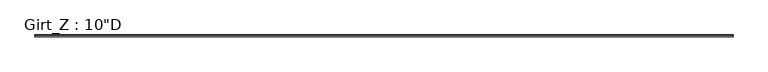
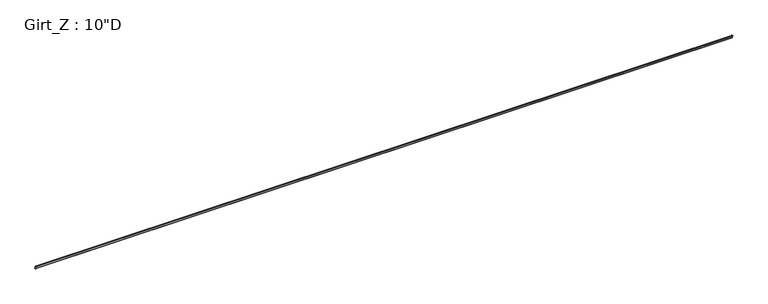
"""IFC4 building model written with IfcOpenShell, lengths in millimetres: beam geometry."""

from ifc_helpers import new_model, si_unit, point, frame, frame_2d, origin, place, context, project, spatial, polyline, circle_curve, trimmed, segment, composite_curve, outline, extrude, source, transform, mapped, element, save


def beam_7a59761d(model_context):
    return source(origin(), model_context, "Body", "SweptSolid", [
        extrude(outline(composite_curve([segment(polyline([(-77.9859375, 127.0), (-3.3734375, 127.0)]), True, "CONTINUOUS"), segment(trimmed(circle_curve(frame_2d((-3.3734375, 122.2375)), 4.7625), [point((-3.3734375, 127.0))], [point((1.3890625, 122.2375))], False, "CARTESIAN"), True, "CONTINUOUS"), segment(polyline([(1.3890625, 122.2375), (1.3890625, -122.2389339)]), True, "CONTINUOUS"), segment(trimmed(circle_curve(frame_2d((3.3748024, -122.2389339)), 1.9857399), [point((1.3890625, -122.2389339))], [point((3.2694106, -124.221875))], True, "CARTESIAN"), True, "CONTINUOUS"), segment(polyline([(3.2694106, -124.221875), (83.0404765, -124.221875), (94.4528742, -110.621109), (96.5810415, -112.4068534), (84.3359375, -127.0), (-1.3890625, -127.0), (-1.3890625, 122.2381931)]), True, "CONTINUOUS"), segment(trimmed(circle_curve(frame_2d((-3.3741066, 122.2381931)), 1.9850441), [point((-1.3890625, 122.2381931))], [point((-3.3005807, 124.221875))], True, "CARTESIAN"), True, "CONTINUOUS"), segment(polyline([(-3.3005807, 124.221875), (-76.6904765, 124.221875), (-88.1028742, 110.621109), (-90.2310415, 112.4068534), (-77.9859375, 127.0)]), True, "CONTINUOUS")], self_intersect=False)), frame((-36640.8081, 0.0, 0.0), z_axis=(1.0, 0.0, 0.0), x_axis=(0.0, 1.0, 0.0)), (0.0, 0.0, 1.0), 73329.038),
    ])


if __name__ == "__main__":
    model = new_model("IFC4")
    model_context = context("Model", 3, world=origin())
    ifc_project = project(units=[si_unit("LENGTHUNIT", "METRE", prefix="MILLI")], contexts=[model_context])
    site = spatial("IfcSite", under=ifc_project)
    building = spatial("IfcBuilding", under=site)
    placement = place(None, origin())
    beam_shape = beam_7a59761d(model_context)
    element("IfcBeam", 1, ObjectType="Girt_Z : 10\"D", at=placement, inside=building, context=model_context, shape_type="MappedRepresentation", body=[
        mapped(beam_shape, transform((0.0, 0.0, 0.0), x_axis=(1.0, 0.0, 0.0), y_axis=(0.0, 1.0, 0.0), z_axis=(0.0, 0.0, 1.0))),
    ])
    save(model, "model.ifc")

# Revit data of these elements
# Type "Girt_Z : 10\"D"
#   half leg = 0' - 1 11/16"
#   Web_Thickness = 0' - 0 7/64"
#   Length [instance default] = 10' - 0"
#   Leg_2 = 0' - 3 3/8"
#   Leg_1 = 0' - 3 1/8"
#   Height = 0' - 10"
#   Structural Material [instance default] = none
# Element 1 (IfcBeam, "Girt_Z : 10\"D")
#   Structural Material = STRUCTURAL STEEL - SEE STRUCT. DWGS
#   Materials on its faces: "STRUCTURAL STEEL - SEE STRUCT. DWGS"
# Materials
#   "STRUCTURAL STEEL - SEE STRUCT. DWGS": class "Metal", colour RGB 137 146 153, transparency 0, Description = "Steel, mill finish", Cost = 0
